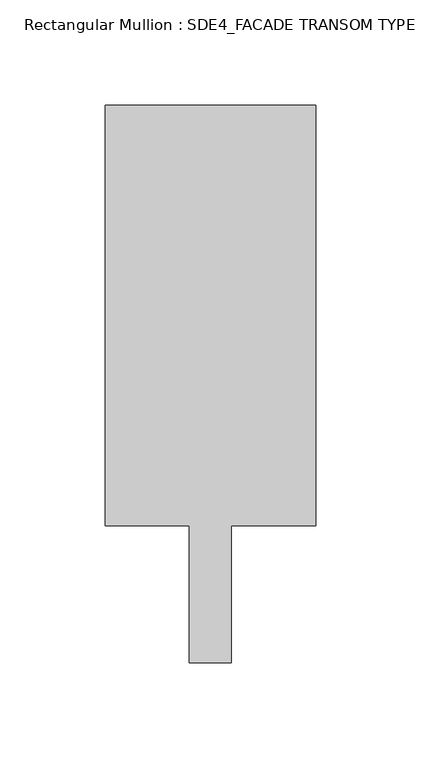
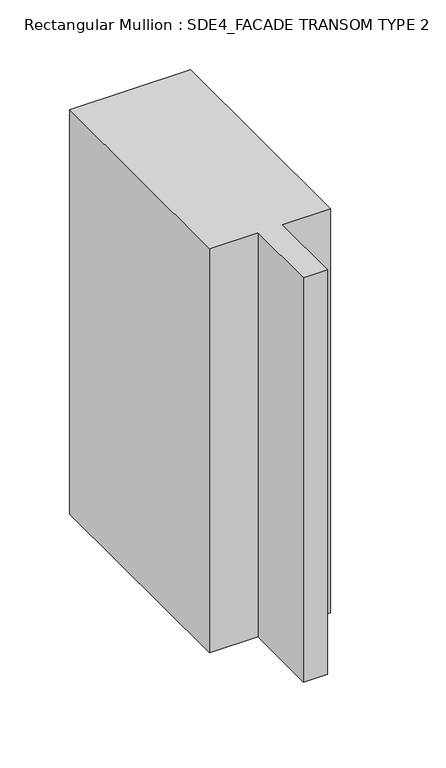
"""IFC4 building model written with IfcOpenShell, lengths in millimetres: member geometry, Rectangular Mullion : SDE4_FACADE TRANSOM TYPE 2."""

from ifc_helpers import new_model, si_unit, frame, origin, place, context, project, spatial, polyline, outline, extrude, source, transform, mapped, element, save


def rectangular_mullion_sde4_facade_transom_type_2_3d03495e(model_context):
    return source(origin(), model_context, "Body", "SweptSolid", [
        extrude(outline(polyline([(50.0, 132.5), (50.0, -67.5), (10.0, -67.5), (10.0, -132.5), (-10.0, -132.5), (-10.0, -67.5), (-50.0, -67.5), (-50.0, 132.5), (50.0, 132.5)])), frame((0.0, 0.0, -352.9472212), z_axis=(0.0, 0.0, 1.0), x_axis=(1.0, 0.0, 0.0)), (0.0, 0.0, 1.0), 352.9472212),
    ])


if __name__ == "__main__":
    model = new_model("IFC4")
    model_context = context("Model", 3, world=origin())
    ifc_project = project(units=[si_unit("LENGTHUNIT", "METRE", prefix="MILLI")], contexts=[model_context])
    site = spatial("IfcSite", under=ifc_project)
    building = spatial("IfcBuilding", under=site)
    placement = place(None, origin())
    rectangular_mullion_sde4_facade_transom_type_2_shape = rectangular_mullion_sde4_facade_transom_type_2_3d03495e(model_context)
    element("IfcMember", 1, ObjectType="Rectangular Mullion : SDE4_FACADE TRANSOM TYPE 2", at=placement, inside=building, context=model_context, shape_type="MappedRepresentation", body=[
        mapped(rectangular_mullion_sde4_facade_transom_type_2_shape, transform((0.0, 0.0, 0.0), x_axis=(1.0, 0.0, 0.0), y_axis=(0.0, 1.0, 0.0), z_axis=(0.0, 0.0, 1.0))),
    ])
    save(model, "model.ifc")

# Revit data of these elements
# Type "Rectangular Mullion : SDE4_FACADE TRANSOM TYPE 2"
#   built-in parameter 1007322 = 0.869423 (stored number, unit not read)
#   built-in parameter 1007321 = 0.164042 (stored number, unit not read)
#   built-in parameter 1007320 = 0.164042 (stored number, unit not read)
